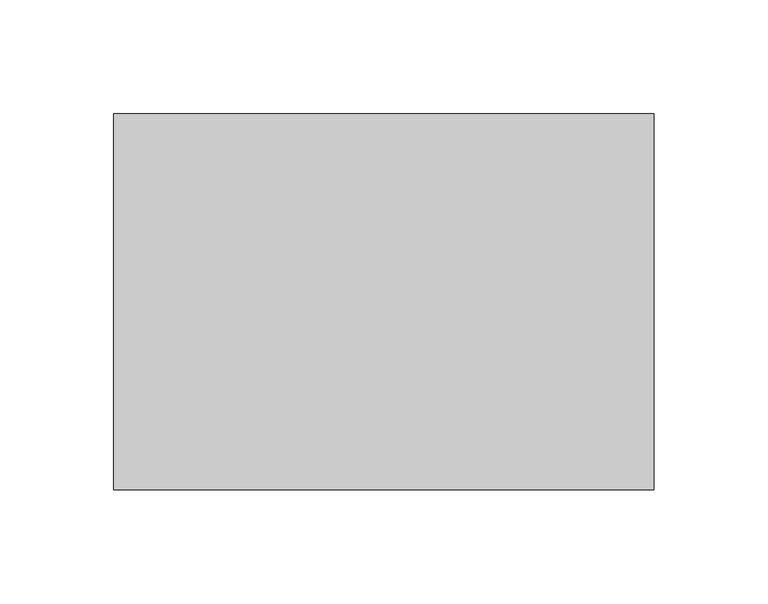
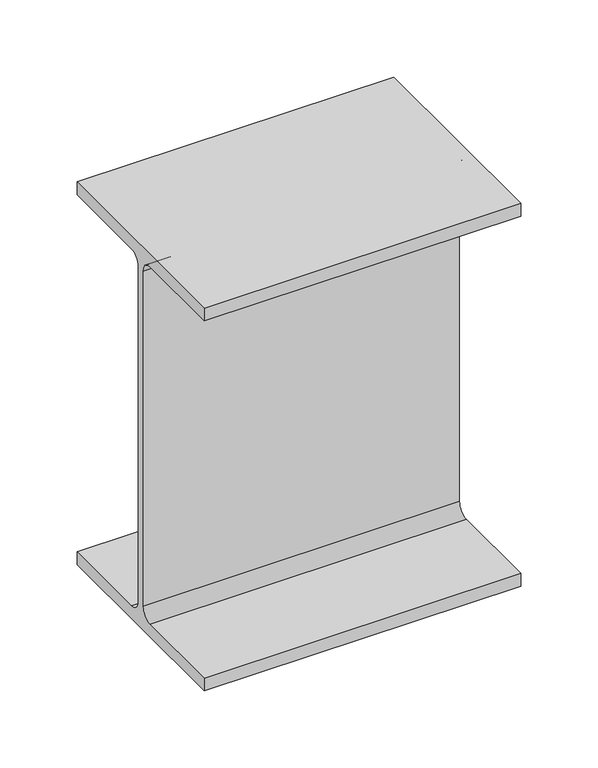
"""IFC4 building model written with IfcOpenShell, lengths in millimetres: beam geometry, Old_Steel Beam_H-KSD3502 : H_SB_ASB_H-300×150x6.5x9."""

from ifc_helpers import new_model, si_unit, point, frame, frame_2d, origin, place, context, project, spatial, polyline, circle_curve, trimmed, segment, composite_curve, outline, extrude, source, transform, mapped, element, save


def beam_1c93ef3f(model_context):
    return source(origin(), model_context, "Body", "SweptSolid", [
        extrude(outline(composite_curve([segment(polyline([(82.5, -141.5), (82.5, -151.7), (-82.5, -151.7), (-82.5, -141.5), (-11.9, -141.5)]), True, "CONTINUOUS"), segment(trimmed(circle_curve(frame_2d((-11.9, -132.6)), 8.9), [point((-11.9, -141.5))], [point((-3.0, -132.6))], True, "CARTESIAN"), True, "CONTINUOUS"), segment(polyline([(-3.0, -132.6), (-3.0, 132.6)]), True, "CONTINUOUS"), segment(trimmed(circle_curve(frame_2d((-11.9, 132.6)), 8.9), [point((-3.0, 132.6))], [point((-11.9, 141.5))], True, "CARTESIAN"), True, "CONTINUOUS"), segment(polyline([(-11.9, 141.5), (-82.5, 141.5), (-82.5, 151.7), (82.5, 151.7), (82.5, 141.5), (11.9, 141.5)]), True, "CONTINUOUS"), segment(trimmed(circle_curve(frame_2d((11.9, 132.6)), 8.9), [point((11.9, 141.5))], [point((3.0, 132.6))], True, "CARTESIAN"), True, "CONTINUOUS"), segment(polyline([(3.0, 132.6), (3.0, -132.6)]), True, "CONTINUOUS"), segment(trimmed(circle_curve(frame_2d((11.9, -132.6)), 8.9), [point((3.0, -132.6))], [point((11.9, -141.5))], True, "CARTESIAN"), True, "CONTINUOUS"), segment(polyline([(11.9, -141.5), (82.5, -141.5)]), True, "CONTINUOUS")], self_intersect=False)), frame((-37.3, 0.0, 0.0), z_axis=(1.0, 0.0, 0.0), x_axis=(0.0, 1.0, 0.0)), (0.0, 0.0, 1.0), 237.2999994),
    ])


if __name__ == "__main__":
    model = new_model("IFC4")
    model_context = context("Model", 3, world=origin())
    ifc_project = project(units=[si_unit("LENGTHUNIT", "METRE", prefix="MILLI")], contexts=[model_context])
    site = spatial("IfcSite", under=ifc_project)
    building = spatial("IfcBuilding", under=site)
    placement = place(None, origin())
    beam_shape = beam_1c93ef3f(model_context)
    element("IfcBeam", 1, ObjectType="Old_Steel Beam_H-KSD3502 : H_SB_ASB_H-300×150x6.5x9", at=placement, inside=building, context=model_context, shape_type="MappedRepresentation", body=[
        mapped(beam_shape, transform((0.0, 0.0, 0.0), x_axis=(1.0, 0.0, 0.0), y_axis=(0.0, 1.0, 0.0), z_axis=(0.0, 0.0, 1.0))),
    ])
    save(model, "model.ifc")

# Revit data of these elements
# Type "Old_Steel Beam_H-KSD3502 : H_SB_ASB_H-300×150x6.5x9"
#   Width = 15.0 cm
#   Web Thickness = 0.65 cm
#   Web Fillet = 1.3 cm
#   Warping Constant = 107174.0 cm⁶
#   Torsional Moment of Inertia = 9.9539 cm⁴
#   Torsional Modulus = 1.0 cm³
#   Section Area = 46.78 cm²
#   Plastic Modulus weak axis = 105.0 cm³
#   Plastic Modulus strong axis = 542.0 cm³
#   Perimeter = 1.17 m²/m
#   Nominal Weight = 36.70 kgf/m
#   Moment of Inertia weak axis = 508.00 cm⁴
#   Moment of Inertia strong axis = 7210.00 cm⁴
#   Height = 30.0 cm
#   Flange Thickness = 0.9 cm
#   Elastic Modulus weak axis = 67.7 cm³
#   Elastic Modulus strong axis = 481.0 cm³
#   Centroid Vertical = 15.0 cm
#   Centroid Horizontal = 7.5 cm
#   Length [instance default] = 1.5240 m
#   Structural Material [instance default] = Steel, 45-345
#   Assembly Code = ""
# Element 1 (IfcBeam, "Old_Steel Beam_H-KSD3502 : H_SB_ASB_H-300×150x6.5x9")
#   Structural Material = none
# Materials
#   "Steel, 45-345": class "Metal", colour RGB 189 187 185, transparency 0, Description = "Steel 345 MPa", Cost = 0
